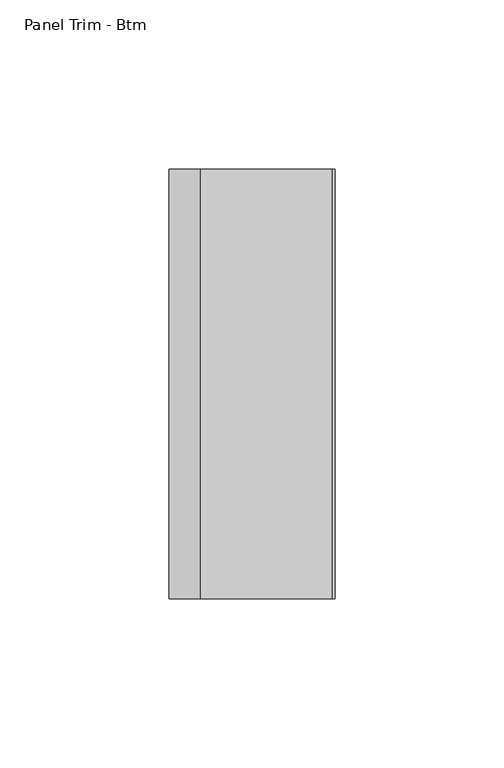
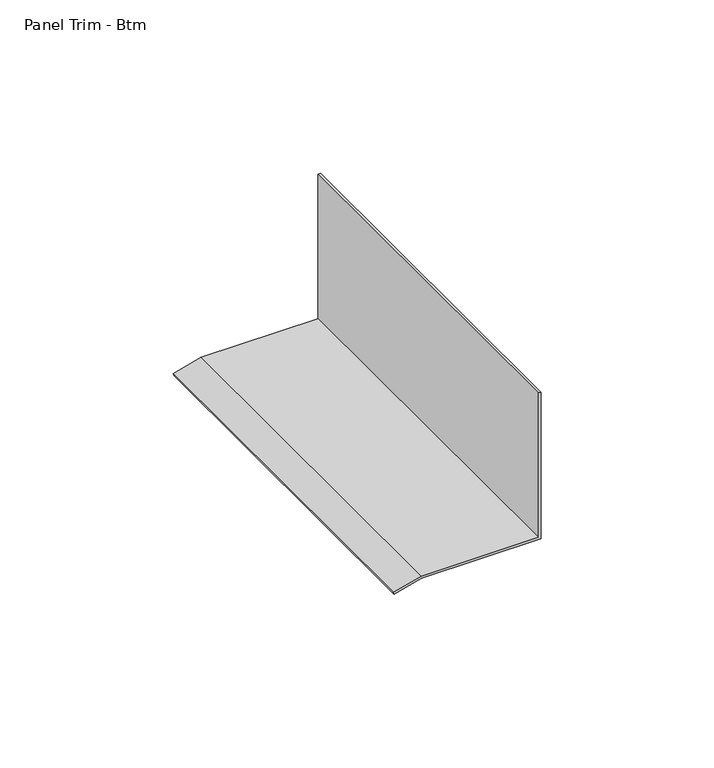
"""IFC4 building model written with IfcOpenShell, lengths in millimetres: proxy geometry, Btm Trim - Mull2 : Panel Trim - Btm."""

from ifc_helpers import new_model, si_unit, frame, origin, place, context, project, spatial, polyline, outline, extrude, source, transform, mapped, element, save


def panel_trim_btm_a4ea7572(model_context):
    return source(origin(), model_context, "Body", "SweptSolid", [
        extrude(outline(polyline([(12.7, 587326.1141748), (10.2077022, 587316.8127928), (9.4409986, 587317.0182304), (11.90625, 587326.2186739), (11.90625, 587365.8934739), (63.5, 587365.8934739), (63.5, 587365.1060739), (12.7, 587365.1060739), (12.7, 587326.1141748)])), frame((0.0, -536420.7663841, 0.0), z_axis=(0.0, 1.0, 0.0), x_axis=(0.0, 0.0, 1.0)), (0.0, 0.0, 1.0), 127.0),
    ])


if __name__ == "__main__":
    model = new_model("IFC4")
    model_context = context("Model", 3, world=origin())
    ifc_project = project(units=[si_unit("LENGTHUNIT", "METRE", prefix="MILLI")], contexts=[model_context])
    site = spatial("IfcSite", under=ifc_project)
    building = spatial("IfcBuilding", under=site)
    placement = place(None, origin())
    panel_trim_btm_shape = panel_trim_btm_a4ea7572(model_context)
    element("IfcBuildingElementProxy", 1, Name="Btm Trim - Mull2 : Panel Trim - Btm", ObjectType="Btm Trim - Mull2 : Panel Trim - Btm", at=placement, inside=building, context=model_context, shape_type="MappedRepresentation", body=[
        mapped(panel_trim_btm_shape, transform((0.0, 0.0, 0.0), x_axis=(1.0, 0.0, 0.0), y_axis=(0.0, 1.0, 0.0), z_axis=(0.0, 0.0, 1.0))),
    ])
    save(model, "model.ifc")

# Revit data of these elements
# Element 1 (IfcBuildingElementProxy, "Btm Trim - Mull2 : Panel Trim - Btm")
#   Materials on its faces: "BASE TRIM BY MTL PANEL MFR."
# Materials
#   "BASE TRIM BY MTL PANEL MFR.": class "Generic", colour RGB 239 242 240, transparency 0, Cost = 0
